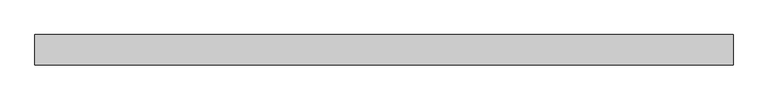
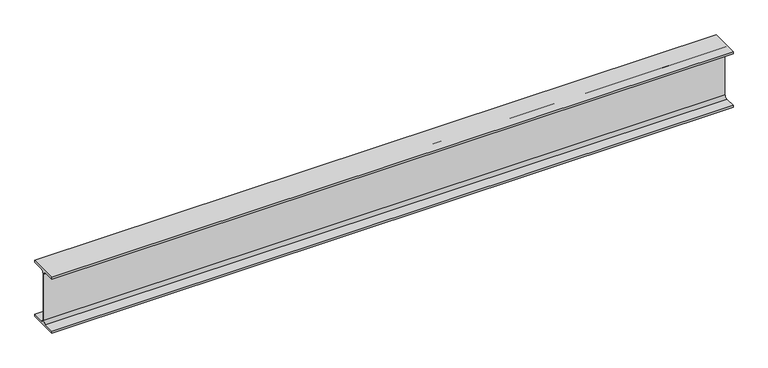
"""IFC4 building model written with IfcOpenShell, lengths in millimetres: beam geometry, 0912_Steel Framing_H-KSD3502 : H_SB_ASB_H-250x125x6x9."""

from ifc_helpers import new_model, si_unit, point, frame, frame_2d, origin, place, context, project, spatial, polyline, circle_curve, trimmed, segment, composite_curve, outline, extrude, source, transform, mapped, element, save


def beam_eb669900(model_context):
    return source(origin(), model_context, "Body", "SweptSolid", [
        extrude(outline(composite_curve([segment(polyline([(62.5, -116.0), (62.5, -125.0), (-62.5, -125.0), (-62.5, -116.0), (-15.0, -116.0)]), True, "CONTINUOUS"), segment(trimmed(circle_curve(frame_2d((-15.0, -104.0)), 12.0), [point((-15.0, -116.0))], [point((-3.0, -104.0))], True, "CARTESIAN"), True, "CONTINUOUS"), segment(polyline([(-3.0, -104.0), (-3.0, 104.0)]), True, "CONTINUOUS"), segment(trimmed(circle_curve(frame_2d((-15.0, 104.0)), 12.0), [point((-3.0, 104.0))], [point((-15.0, 116.0))], True, "CARTESIAN"), True, "CONTINUOUS"), segment(polyline([(-15.0, 116.0), (-62.5, 116.0), (-62.5, 125.0), (62.5, 125.0), (62.5, 116.0), (15.0, 116.0)]), True, "CONTINUOUS"), segment(trimmed(circle_curve(frame_2d((15.0, 104.0)), 12.0), [point((15.0, 116.0))], [point((3.0, 104.0))], True, "CARTESIAN"), True, "CONTINUOUS"), segment(polyline([(3.0, 104.0), (3.0, -104.0)]), True, "CONTINUOUS"), segment(trimmed(circle_curve(frame_2d((15.0, -104.0)), 12.0), [point((3.0, -104.0))], [point((15.0, -116.0))], True, "CARTESIAN"), True, "CONTINUOUS"), segment(polyline([(15.0, -116.0), (62.5, -116.0)]), True, "CONTINUOUS")], self_intersect=False)), frame((-1404.8, 0.0, 0.0), z_axis=(1.0, 0.0, 0.0), x_axis=(0.0, 1.0, 0.0)), (0.0, 0.0, 1.0), 2892.0999994),
    ])


if __name__ == "__main__":
    model = new_model("IFC4")
    model_context = context("Model", 3, world=origin())
    ifc_project = project(units=[si_unit("LENGTHUNIT", "METRE", prefix="MILLI")], contexts=[model_context])
    site = spatial("IfcSite", under=ifc_project)
    building = spatial("IfcBuilding", under=site)
    placement = place(None, origin())
    beam_shape = beam_eb669900(model_context)
    element("IfcBeam", 1, ObjectType="0912_Steel Framing_H-KSD3502 : H_SB_ASB_H-250x125x6x9", at=placement, inside=building, context=model_context, shape_type="MappedRepresentation", body=[
        mapped(beam_shape, transform((0.0, 0.0, 0.0), x_axis=(1.0, 0.0, 0.0), y_axis=(0.0, 1.0, 0.0), z_axis=(0.0, 0.0, 1.0))),
    ])
    save(model, "model.ifc")

# Revit data of these elements
# Type "0912_Steel Framing_H-KSD3502 : H_SB_ASB_H-250x125x6x9"
#   H_WM Code_1 = "S01AA003-00001 | Main Steel Structure Fabrication Work | Shelter/Building | Light Steel - Standard (30KG/M>Weight) | Material: (   )"
#   H_WM Code_2 = "S03AA029-00001 | Main Steel Structure Erection Work | Shelter/Building | Light Steel (30KG/M>Weight) | Material: (   )"
#   H_WM Code_3 = "S01AA010-00001 | Main Steel Structure Fabrication Work | Shelter/Building | Steel Painting/Coating | for Non-Fireproofed Steel Surface, Surface Preparation, Primer, Second & Final Coat | Material: (   )"
#   H_Q'ty Cal Type Tag = "SB-Q2"
#   Width = 12.5 cm
#   Web Thickness = 0.6 cm
#   Web Fillet = 1.2 cm
#   Warping Constant = 42539.8 cm⁶
#   W = 0
#   Torsional Moment of Inertia = 7.8102 cm⁴
#   Section Area = 37.66 cm²
#   Plastic Modulus weak axis = 73.1 cm³
#   Plastic Modulus strong axis = 366.0 cm³
#   Perimeter = 0.97 m²/m
#   Nominal Weight = 29.60 kgf/m
#   Moment of Inertia weak axis = 294.00 cm⁴
#   Moment of Inertia strong axis = 4050.00 cm⁴
#   Height = 25.0 cm
#   Flange Thickness = 0.9 cm
#   Elastic Modulus weak axis = 47.0 cm³
#   Elastic Modulus strong axis = 324.0 cm³
#   Centroid Vertical = 12.5 cm
#   Centroid Horizontal = 6.25 cm
#   Ix = 40500000
#   Length [instance default] = 1.5240 m
#   Zx = 366000
#   b = 0.1250 m
#   h = 0.2500 m
#   r = 0.0120 m
#   s = 0.0060 m
#   t = 0.0090 m
#   A = 0.003766 m²
#   Structural Material [instance default] = Steel, 45-345
#   Assembly Code = ""
# Element 1 (IfcBeam, "0912_Steel Framing_H-KSD3502 : H_SB_ASB_H-250x125x6x9")
#   Structural Material = none
# Materials
#   "Steel, 45-345": class "Metal", colour RGB 189 187 185, transparency 0, Description = "Steel 345 MPa", Cost = 0
